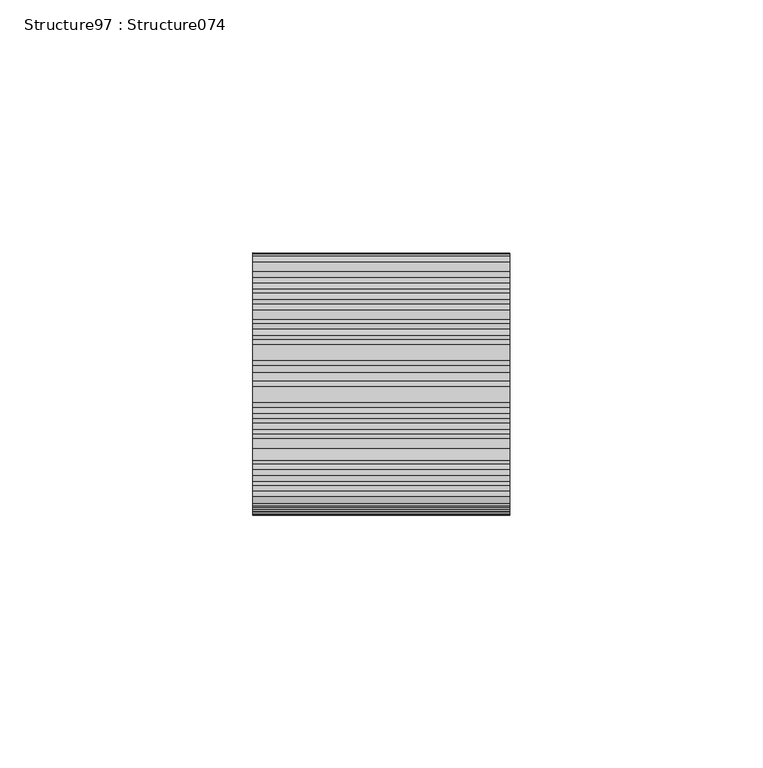
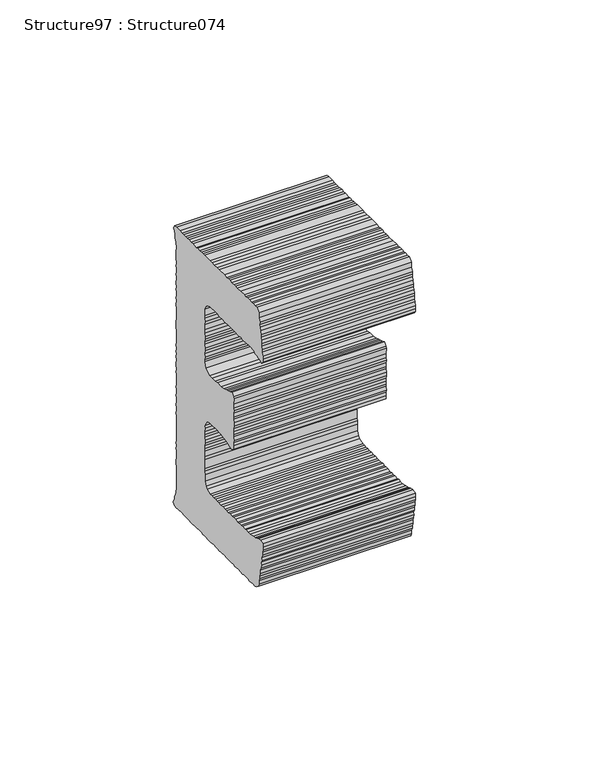
"""IFC4 building model written with IfcOpenShell, lengths in millimetres: proxy geometry, Structure97 : Structure074."""

import ifcopenshell
import ifcopenshell.guid

model = None  # the IFC model being written
_history = None  # IfcOwnerHistory: only IFC2X3 demands one
_inside = {}  # id of a spatial element -> (the spatial element, [elements in it])
_under = {}  # id of a project, library or spatial element -> (it, [spatial elements below it])
_declared = {}  # id of a project -> (the project, [libraries it declares])
_typed = {}  # id of a type object -> (the type object, [elements of that type])
_made_of = {}  # id of a material, layer set ... -> (it, [elements and type objects made of it])


def new_model(schema):
    """Start an empty IFC model of exactly this schema.

    Asked for "IFC4X3", IfcOpenShell would pick the latest addendum, in which some entities
    have other attributes; the version numbers below select the first issue.
    IFC2X3 requires an IfcOwnerHistory on every rooted entity: one is made here for all.
    """
    global model, _history
    if schema == "IFC4X3":
        model = ifcopenshell.file(schema_version=(4, 3, 0, 0))
    else:
        model = ifcopenshell.file(schema=schema)
    _inside.clear()
    _under.clear()
    _declared.clear()
    _typed.clear()
    _made_of.clear()
    _history = None
    if model.schema == "IFC2X3":
        org = make("IfcOrganization", Name="unknown")
        user = make(
            "IfcPersonAndOrganization",
            ThePerson=make("IfcPerson", FamilyName="unknown"),
            TheOrganization=org,
        )
        app = make(
            "IfcApplication",
            ApplicationDeveloper=org,
            Version="unknown",
            ApplicationFullName="unknown",
            ApplicationIdentifier="unknown",
        )
        _history = make(
            "IfcOwnerHistory",
            OwningUser=user,
            OwningApplication=app,
            ChangeAction="ADDED",
            CreationDate=0,
        )
    return model


def make(cls, **values):
    """One entity of the class cls with the attributes given. An attribute that is None is left unset."""
    return model.create_entity(
        cls, **{name: value for name, value in values.items() if value is not None}
    )


def rooted(cls, **values):
    """An entity with a GlobalId (a new one), such as an element, a storey or a relation."""
    return make(cls, GlobalId=ifcopenshell.guid.new(), OwnerHistory=_history, **values)


def si_unit(unit_type, name, prefix=None):
    """IfcSIUnit, for example si_unit("LENGTHUNIT", "METRE", prefix="MILLI")."""
    return make("IfcSIUnit", UnitType=unit_type, Prefix=prefix, Name=name)


def assignment(units):
    """IfcUnitAssignment: the units of a project."""
    return None if units is None else make("IfcUnitAssignment", Units=units)


def point(xyz):
    """IfcCartesianPoint."""
    return None if xyz is None else make("IfcCartesianPoint", Coordinates=xyz)


def direction(xyz):
    """IfcDirection."""
    return None if xyz is None else make("IfcDirection", DirectionRatios=xyz)


def frame(location, z_axis=None, x_axis=None):
    """IfcAxis2Placement3D, a coordinate frame: its origin and axes. An axis left out is left unset."""
    return make(
        "IfcAxis2Placement3D",
        Location=point(location),
        Axis=direction(z_axis),
        RefDirection=direction(x_axis),
    )


def origin():
    """The frame at (0, 0, 0) with its axes left unset."""
    return frame((0.0, 0.0, 0.0))


def place(relative_to, where):
    """IfcLocalPlacement: puts the frame where relative to a parent placement (None: the world)."""
    return make(
        "IfcLocalPlacement", PlacementRelTo=relative_to, RelativePlacement=where
    )


def context(
    kind, dimensions, precision=None, world=None, true_north=None, identifier=None
):
    """IfcGeometricRepresentationContext, for example the 3D "Model" context."""
    return make(
        "IfcGeometricRepresentationContext",
        ContextIdentifier=identifier,
        ContextType=kind,
        CoordinateSpaceDimension=dimensions,
        Precision=precision,
        WorldCoordinateSystem=world,
        TrueNorth=true_north,
    )


def project(units=None, contexts=None):
    """IfcProject with its units and contexts."""
    return rooted(
        "IfcProject",
        Name="project",
        RepresentationContexts=contexts,
        UnitsInContext=assignment(units),
    )


def spatial(cls, under=None, at=None, **own):
    """A site, building, storey or space (cls), placed at a placement, below another one or the project."""
    s = rooted(cls, ObjectPlacement=at, **own)
    if under is not None:
        _under.setdefault(under.id(), (under, []))[1].append(s)
    return s


def polyline(points):
    """IfcPolyline through the points."""
    return make("IfcPolyline", Points=[point(p) for p in points])


def outline(outer, holes=None, kind="AREA"):
    """IfcArbitraryClosedProfileDef: a profile drawn as a closed curve; with holes, ...WithVoids."""
    if holes is None:
        return make("IfcArbitraryClosedProfileDef", ProfileType=kind, OuterCurve=outer)
    return make(
        "IfcArbitraryProfileDefWithVoids",
        ProfileType=kind,
        OuterCurve=outer,
        InnerCurves=holes,
    )


def extrude(swept, where, along, depth):
    """IfcExtrudedAreaSolid: the profile swept, set in the frame where, extruded along a direction by depth."""
    return make(
        "IfcExtrudedAreaSolid",
        SweptArea=swept,
        Position=where,
        ExtrudedDirection=direction(along),
        Depth=depth,
    )


def shape(context_of_items, identifier, shape_type, items):
    """IfcShapeRepresentation: the items that make up one representation, for example the "Body"."""
    return make(
        "IfcShapeRepresentation",
        ContextOfItems=context_of_items,
        RepresentationIdentifier=identifier,
        RepresentationType=shape_type,
        Items=items,
    )


def source(mapping_origin, context_of_items, identifier, shape_type, items):
    """IfcRepresentationMap: a shape defined once, which mapped items show again and again."""
    return make(
        "IfcRepresentationMap",
        MappingOrigin=mapping_origin,
        MappedRepresentation=shape(context_of_items, identifier, shape_type, items),
    )


def transform(
    local_origin,
    x_axis=None,
    y_axis=None,
    z_axis=None,
    scale=None,
    scale2=None,
    scale3=None,
    uniform=True,
):
    """IfcCartesianTransformationOperator3D, or its non-uniform kind. x_axis, y_axis, z_axis: its Axis1, 2, 3."""
    if uniform:
        return make(
            "IfcCartesianTransformationOperator3D",
            Axis1=direction(x_axis),
            Axis2=direction(y_axis),
            LocalOrigin=point(local_origin),
            Scale=scale,
            Axis3=direction(z_axis),
        )
    return make(
        "IfcCartesianTransformationOperator3DnonUniform",
        Axis1=direction(x_axis),
        Axis2=direction(y_axis),
        LocalOrigin=point(local_origin),
        Scale=scale,
        Axis3=direction(z_axis),
        Scale2=scale2,
        Scale3=scale3,
    )


def mapped(mapping_source, mapping_target):
    """IfcMappedItem: shows the shape of a source again, moved by a transform."""
    return make(
        "IfcMappedItem", MappingSource=mapping_source, MappingTarget=mapping_target
    )


def made_of(thing, what):
    """Note that an element or type object is made of a material, layer set ...; save() writes the relation."""
    if what is not None:
        _made_of.setdefault(what.id(), (what, []))[1].append(thing)
    return thing


def element(
    cls,
    number,
    at=None,
    inside=None,
    cuts=None,
    type_object=None,
    material=None,
    context=None,
    identifier="Body",
    shape_type=None,
    held_by="IfcProductDefinitionShape",
    body=None,
    shapes=None,
    **own,
):
    """One element of the class cls, such as IfcWall. Its Tag is "e" and its number.

    at: its placement. inside: the storey or other place that contains it. cuts: it is an
    opening in that element (IfcRelVoidsElement). A single representation is given by context,
    identifier, shape_type and body (its items); several are given by shapes. held_by: the class
    of the entity that holds the representations. save() writes the other relations.
    """
    e = rooted(cls, Tag="e%d" % number, ObjectPlacement=at, **own)
    if body is not None:
        shapes = [shape(context, identifier, shape_type, body)]
    if shapes is not None:
        e.Representation = make(held_by, Representations=shapes)
    if inside is not None:
        _inside.setdefault(inside.id(), (inside, []))[1].append(e)
    if cuts is not None:
        rooted(
            "IfcRelVoidsElement", RelatingBuildingElement=cuts, RelatedOpeningElement=e
        )
    if type_object is not None:
        _typed.setdefault(type_object.id(), (type_object, []))[1].append(e)
    return made_of(e, material)


def aggregate(whole, parts):
    """IfcRelAggregates: a whole, such as a stair, and the parts it consists of."""
    return rooted("IfcRelAggregates", RelatingObject=whole, RelatedObjects=parts)


def save(model, path):
    """Write the relations noted so far, then the file.

    IfcRelAggregates (storeys below a building ...), IfcRelContainedInSpatialStructure (elements
    in a storey), IfcRelDefinesByType, IfcRelAssociatesMaterial and IfcRelDeclares: one each for
    every whole, place, type object, material and project.
    """
    for whole, parts in _under.values():
        aggregate(whole, parts)
    for where, things in _inside.values():
        rooted(
            "IfcRelContainedInSpatialStructure",
            RelatedElements=things,
            RelatingStructure=where,
        )
    for kind, things in _typed.values():
        rooted("IfcRelDefinesByType", RelatedObjects=things, RelatingType=kind)
    for what, things in _made_of.values():
        rooted("IfcRelAssociatesMaterial", RelatedObjects=things, RelatingMaterial=what)
    for by, libraries in _declared.values():
        rooted("IfcRelDeclares", RelatingContext=by, RelatedDefinitions=libraries)
    model.write(path)


def structure97_structure074_eda54e12(model_context):
    return source(origin(), model_context, "Body", "SweptSolid", [
        extrude(outline(polyline([(1.48162, 0.0), (2.2572371, -0.2724071), (3.0991635, -1.0956216), (4.9019403, -2.1639485), (5.4589512, -2.9293375), (7.3048622, -4.363736), (8.081852, -4.6349566), (9.0300726, -5.5353617), (9.7680435, -6.2777957), (10.5884483, -6.9153062), (11.4674269, -7.2657789), (12.1278313, -8.1115116), (13.031513, -8.6447535), (15.4930086, -10.5575032), (16.0253163, -11.140123), (17.6686547, -12.4171088), (18.7521725, -12.9265225), (19.3904936, -13.5861146), (20.2123032, -14.2247167), (21.0525437, -15.0466212), (21.7502814, -15.4198305), (22.753051, -16.0354777), (23.4711862, -16.5935177), (25.1576587, -18.2365751), (25.9576659, -18.6892549), (26.6956368, -19.4316889), (29.8766723, -21.9035703), (30.8579205, -22.3335134), (31.6783254, -22.9710239), (32.3384489, -23.8165383), (33.1384561, -24.2692181), (33.8781127, -25.012962), (34.9840861, -25.7033983), (35.6203492, -26.3667985), (37.2636876, -27.6437843), (38.2676722, -28.2549685), (39.0894819, -28.8935705), (38.9651916, -30.1100787), (37.6526818, -30.742572), (36.993088, -31.3768362), (35.9689867, -32.0626598), (35.0198928, -32.6449986), (33.7000538, -33.9224837), (32.9604919, -34.6631371), (32.3473089, -35.6633154), (31.6837244, -36.3061945), (30.4067385, -37.9495329), (29.873026, -38.8474416), (29.1334642, -39.5880949), (28.701522, -40.5655367), (27.9825762, -41.4907398), (27.3251674, -42.1262514), (26.5015502, -42.9750746), (25.8883673, -43.9752529), (25.4288228, -44.7771356), (24.6908519, -45.5163216), (24.1555485, -46.4156976), (23.3934684, -46.9748293), (22.8595376, -47.8730188), (22.1429933, -48.7951314), (21.4805003, -49.4366057), (20.8432082, -50.2567296), (20.2300253, -51.2569079), (19.4880618, -52.0006518), (18.9530394, -52.9002463), (18.2905464, -53.5417206), (17.7782605, -54.6225558), (16.9608192, -55.4640114), (16.3764867, -56.0049019), (15.944763, -56.9820627), (15.0213404, -57.7488241), (14.4863179, -58.6484185), (13.8730723, -59.6480975), (13.1902444, -60.1052404), (12.5733499, -61.110195), (12.1210101, -61.9028061), (11.1943126, -62.6737819), (10.6606001, -63.5716906), (9.3860159, -65.2119383), (8.7701503, -66.2149889), (8.0862308, -66.6735366), (7.4933827, -67.8580463), (6.9377444, -68.5730909), (6.1144082, -69.4221325), (5.5801964, -70.3201037), (4.7425757, -70.9764477), (4.4645531, -71.7558122), (3.5435321, -72.5194831), (3.0301545, -73.6017232), (2.1888223, -74.2628434), (0.9118364, -75.9061818), (0.4560662, -76.7037876), (-0.1801343, -77.5225066), (-0.6359673, -78.3196131), (-1.9943886, -80.0677497), (-2.9140996, -80.8297348), (-4.0071621, -82.4474645), (-4.8283776, -83.293197), (-5.7399809, -84.8879092), (-6.5572039, -85.7290839), (-7.0946906, -86.6312695), (-7.9123503, -87.4730061), (-8.5494242, -88.2928491), (-8.9297165, -88.9927431), (-9.6689973, -89.7336149), (-10.2064841, -90.6358005), (-11.8416478, -92.3184934), (-12.1172688, -93.0947674), (-12.9575094, -93.7544829), (-13.6521278, -94.8594595), (-14.0300185, -95.5562629), (-14.9534411, -96.3230244), (-15.4646354, -97.4024548), (-17.2199725, -99.6613778), (-18.1394652, -100.4230819), (-19.05478, -102.0225704), (-19.2578232, -103.3410046), (-19.8695388, -104.3427738), (-20.3033511, -105.3255216), (-20.5537393, -106.2827232), (-21.4192127, -106.761511), (-22.4259747, -106.1504218), (-23.9642339, -104.9550896), (-24.8064733, -104.1293788), (-25.6263162, -103.4923049), (-26.6316735, -102.8823073), (-27.1645754, -102.2969728), (-28.3531724, -101.7059054), (-28.9096214, -100.9409531), (-29.9152597, -100.3307372), (-31.3716789, -99.0277667), (-32.1483878, -98.7567645), (-32.8090732, -97.9108135), (-33.9945797, -97.3221476), (-34.5322847, -96.7429942), (-35.4302882, -96.2065043), (-37.8937504, -94.2922263), (-38.6354328, -93.5545686), (-39.5782562, -92.6506971), (-40.9952206, -91.7208527), (-41.9968986, -91.1038007), (-44.458956, -89.1906143), (-45.1190795, -88.3450999), (-46.2028783, -87.8354679), (-46.9207325, -87.2776462), (-47.4771816, -86.512694), (-48.5046543, -85.7142776), (-49.3057533, -85.2630026), (-49.9423296, -84.597106), (-51.478622, -83.4033022), (-53.4873429, -82.1749426), (-53.9403985, -81.4903341), (-54.9230514, -81.0592993), (-55.8471308, -80.3412267), (-56.6910827, -79.5240985), (-57.3851089, -79.1461129), (-58.2304657, -78.3278931), (-59.0522754, -77.6892909), (-59.437277, -76.0675653), (-58.3214154, -74.6315759), (-57.9340122, -73.2869709), (-57.2742019, -72.6483688), (-56.8965294, -71.9518463), (-56.56848, -70.8941235), (-55.9773177, -69.7083038), (-55.3156033, -69.0707307), (-54.9631637, -68.1932804), (-54.5269176, -67.2097202), (-53.9725892, -66.4963614), (-53.3575987, -65.4903778), (-52.9805187, -64.7951975), (-52.5729988, -63.6352049), (-52.1137352, -62.8331039), (-51.4766614, -62.013261), (-50.3029742, -61.7739761), (-50.10932, -62.5819051), (-49.2688612, -63.4035286), (-48.6049635, -64.2447659), (-47.8648075, -64.9884473), (-47.6716526, -65.7964387), (-45.9830918, -67.4339091), (-44.3397534, -68.710895), (-43.4642681, -69.0658631), (-42.5421556, -69.7824074), (-41.8782579, -70.6236447), (-40.8988171, -71.0593933), (-40.1809629, -71.617215), (-39.518751, -72.4571423), (-38.4143041, -73.1536022), (-35.9525276, -75.0665702), (-35.0517468, -75.6029653), (-34.3338925, -76.160787), (-33.569411, -77.0801848), (-32.6936448, -77.4353712), (-31.7454241, -78.3357763), (-31.2082183, -78.9149923), (-29.5679706, -80.1895766), (-28.667782, -80.7273138), (-27.8226435, -81.5458146), (-26.091727, -82.0716378), (-24.9148275, -81.8276393), (-23.6088048, -81.2040741), (-22.1744063, -79.3581632), (-21.7967338, -78.6616407), (-21.1851739, -77.6606517), (-20.2581634, -76.8921723), (-19.3224509, -75.4775145), (-18.6067799, -74.5565258), (-17.99522, -73.5555369), (-17.4334685, -72.8326253), (-16.5920415, -72.1742824), (-16.0364031, -71.4592377), (-15.5207188, -70.3711298), (-14.9663903, -69.6577709), (-14.14377, -68.8131299), (-13.6101523, -67.9124439), (-12.7682887, -67.253539), (-12.2864443, -66.6334591), (-11.6033033, -64.6971925), (-12.7339798, -62.3423671), (-13.6792996, -61.4388089), (-15.1169749, -60.3216373), (-16.3013897, -59.7315667), (-17.9444471, -58.4547991), (-19.6194081, -57.6493666), (-20.8856037, -57.1593197), (-21.7611516, -56.8038523), (-22.8446694, -56.2944386), (-23.9836434, -56.0645715), (-24.2452299, -54.7050245), (-23.8705513, -54.0129348), (-22.3881206, -52.5296916), (-21.6973712, -51.4262147), (-21.3167979, -50.7265391), (-20.4777725, -50.0712867), (-19.7844032, -48.9644382), (-19.2020965, -48.4296341), (-18.6883772, -47.3440548), (-17.9731428, -46.423628), (-17.127786, -45.7602278), (-16.4907121, -44.9403848), (-16.0331344, -44.1369737), (-15.3748505, -43.5043954), (-14.8650609, -42.4238733), (-14.0978646, -41.861057), (-13.5658379, -40.9618384), (-12.8492936, -40.0397258), (-11.3397581, -40.2177813), (-10.9453387, -41.1889281), (-10.3872362, -41.9529122), (-9.5147744, -42.9508106), (-8.936523, -43.9016851), (-7.6375485, -45.40495), (-6.8375413, -45.8576298), (-5.8925025, -46.7609697), (-5.3556082, -47.3417462), (-4.1701017, -47.9304121), (-3.5344004, -48.5933756), (-2.6089163, -49.3125398), (-0.8759114, -49.832776), (1.5023395, -48.8888325), (1.7787391, -48.1086572), (2.6760267, -47.1679277), (3.3133188, -46.3478038), (3.9768407, -45.7044254), (4.3255061, -44.8312522), (4.9649815, -44.0083187), (5.8895904, -43.2429299), (6.5268826, -42.4228059), (6.9034634, -41.7276882), (8.0985772, -40.1897101), (8.9184202, -39.3451639), (10.8324798, -36.8819825), (11.2090607, -36.1868648), (11.8208388, -35.185595), (13.1770769, -33.440268), (13.7251051, -31.8883767), (13.7916324, -30.9572831), (12.5728444, -29.3473481), (11.6711294, -28.8156345), (11.2163881, -28.1297161), (10.0308816, -27.5410502), (9.5758593, -26.8549135), (8.6753594, -26.3187367), (7.8308132, -25.4988938), (6.643902, -24.9091362), (5.9832165, -24.0631853), (5.0841214, -23.5281001), (4.4438335, -22.8669798), (3.3620016, -22.3588761), (2.8035858, -21.5923956), (2.0064794, -21.1365626), (1.0008089, -20.5240685), (0.1361462, -19.5196133), (-0.6612412, -19.063562), (-1.4032368, -18.3234078), (-2.2824963, -17.9727167), (-3.1457542, -16.9693531), (-3.922463, -16.6983508), (-4.5831486, -15.8523998), (-5.4046773, -15.214016), (-7.3669551, -14.3538486), (-8.2671437, -13.8161113), (-9.1459038, -13.4653575), (-10.1011405, -13.2124408), (-11.2864608, -12.6212158), (-12.2547033, -11.5389758), (-11.4562869, -10.511503), (-10.8200864, -9.6927839), (-10.1364479, -9.2340179), (-9.2370719, -8.2877013), (-8.2901611, -7.7081721), (-7.8362949, -6.9095374), (-6.8680525, -6.5101574), (-6.3302848, -5.6081901), (-5.40945, -4.8470783), (-4.5434772, -4.3682278), (-3.7463708, -3.3424408), (-2.9842908, -2.7833092), (-2.4264692, -2.0654549), (-1.4788426, -1.4815252), (-0.580245, -0.5391099), (0.0, 0.0), (1.48162, 0.0)])), frame((-56111.2432242, 291863.863217, -374.3014721), z_axis=(-0.9999998917542983, 0.00046528635450596156, 0.0), x_axis=(0.0003674011318705442, 0.7896236125134088, -0.6135914076791513)), (0.0, 0.0, 1.0), 50.8),
    ])


if __name__ == "__main__":
    model = new_model("IFC4")
    model_context = context("Model", 3, world=origin())
    ifc_project = project(units=[si_unit("LENGTHUNIT", "METRE", prefix="MILLI")], contexts=[model_context])
    site = spatial("IfcSite", under=ifc_project)
    building = spatial("IfcBuilding", under=site)
    placement = place(None, origin())
    structure97_structure074_shape = structure97_structure074_eda54e12(model_context)
    element("IfcBuildingElementProxy", 1, Name="Structure97 : Structure074", ObjectType="Structure97 : Structure074", at=placement, inside=building, context=model_context, shape_type="MappedRepresentation", body=[
        mapped(structure97_structure074_shape, transform((0.0, 0.0, 0.0), x_axis=(1.0, 0.0, 0.0), y_axis=(0.0, 1.0, 0.0), z_axis=(0.0, 0.0, 1.0))),
    ])
    save(model, "model.ifc")

# Revit data of these elements
# Type "Structure97 : Structure074"
#   NameOverride = "Structure074"
# Element 1 (IfcBuildingElementProxy, "Structure97 : Structure074")
#   Materials on its faces: "BRUSHED ALUMINUM LETTERING"
# Materials
#   "BRUSHED ALUMINUM LETTERING": class "Unassigned", colour RGB 169 181 186, transparency 0, Cost = 0
